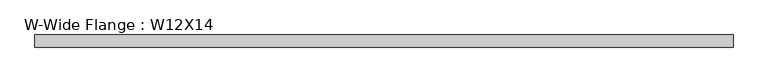
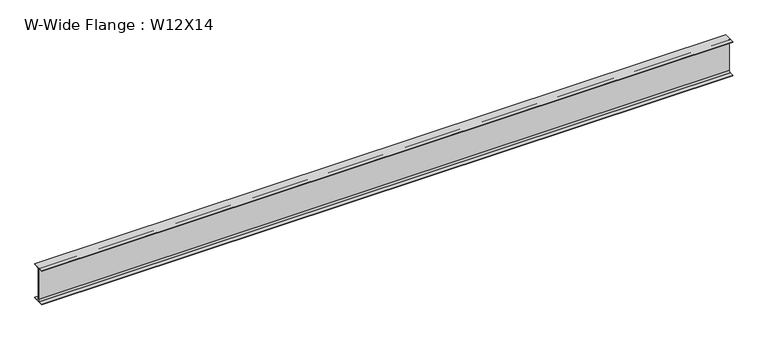
"""IFC4 building model written with IfcOpenShell, lengths in millimetres: beam geometry, W-Wide Flange : W12X14."""

import ifcopenshell
import ifcopenshell.guid

model = None  # the IFC model being written
_history = None  # IfcOwnerHistory: only IFC2X3 demands one
_inside = {}  # id of a spatial element -> (the spatial element, [elements in it])
_under = {}  # id of a project, library or spatial element -> (it, [spatial elements below it])
_declared = {}  # id of a project -> (the project, [libraries it declares])
_typed = {}  # id of a type object -> (the type object, [elements of that type])
_made_of = {}  # id of a material, layer set ... -> (it, [elements and type objects made of it])


def new_model(schema):
    """Start an empty IFC model of exactly this schema.

    Asked for "IFC4X3", IfcOpenShell would pick the latest addendum, in which some entities
    have other attributes; the version numbers below select the first issue.
    IFC2X3 requires an IfcOwnerHistory on every rooted entity: one is made here for all.
    """
    global model, _history
    if schema == "IFC4X3":
        model = ifcopenshell.file(schema_version=(4, 3, 0, 0))
    else:
        model = ifcopenshell.file(schema=schema)
    _inside.clear()
    _under.clear()
    _declared.clear()
    _typed.clear()
    _made_of.clear()
    _history = None
    if model.schema == "IFC2X3":
        org = make("IfcOrganization", Name="unknown")
        user = make(
            "IfcPersonAndOrganization",
            ThePerson=make("IfcPerson", FamilyName="unknown"),
            TheOrganization=org,
        )
        app = make(
            "IfcApplication",
            ApplicationDeveloper=org,
            Version="unknown",
            ApplicationFullName="unknown",
            ApplicationIdentifier="unknown",
        )
        _history = make(
            "IfcOwnerHistory",
            OwningUser=user,
            OwningApplication=app,
            ChangeAction="ADDED",
            CreationDate=0,
        )
    return model


def make(cls, **values):
    """One entity of the class cls with the attributes given. An attribute that is None is left unset."""
    return model.create_entity(
        cls, **{name: value for name, value in values.items() if value is not None}
    )


def rooted(cls, **values):
    """An entity with a GlobalId (a new one), such as an element, a storey or a relation."""
    return make(cls, GlobalId=ifcopenshell.guid.new(), OwnerHistory=_history, **values)


def si_unit(unit_type, name, prefix=None):
    """IfcSIUnit, for example si_unit("LENGTHUNIT", "METRE", prefix="MILLI")."""
    return make("IfcSIUnit", UnitType=unit_type, Prefix=prefix, Name=name)


def assignment(units):
    """IfcUnitAssignment: the units of a project."""
    return None if units is None else make("IfcUnitAssignment", Units=units)


def point(xyz):
    """IfcCartesianPoint."""
    return None if xyz is None else make("IfcCartesianPoint", Coordinates=xyz)


def direction(xyz):
    """IfcDirection."""
    return None if xyz is None else make("IfcDirection", DirectionRatios=xyz)


def frame(location, z_axis=None, x_axis=None):
    """IfcAxis2Placement3D, a coordinate frame: its origin and axes. An axis left out is left unset."""
    return make(
        "IfcAxis2Placement3D",
        Location=point(location),
        Axis=direction(z_axis),
        RefDirection=direction(x_axis),
    )


def frame_2d(location, x_axis=None):
    """IfcAxis2Placement2D, a coordinate frame in the plane: its origin and x axis."""
    return make(
        "IfcAxis2Placement2D", Location=point(location), RefDirection=direction(x_axis)
    )


def origin():
    """The frame at (0, 0, 0) with its axes left unset."""
    return frame((0.0, 0.0, 0.0))


def place(relative_to, where):
    """IfcLocalPlacement: puts the frame where relative to a parent placement (None: the world)."""
    return make(
        "IfcLocalPlacement", PlacementRelTo=relative_to, RelativePlacement=where
    )


def context(
    kind, dimensions, precision=None, world=None, true_north=None, identifier=None
):
    """IfcGeometricRepresentationContext, for example the 3D "Model" context."""
    return make(
        "IfcGeometricRepresentationContext",
        ContextIdentifier=identifier,
        ContextType=kind,
        CoordinateSpaceDimension=dimensions,
        Precision=precision,
        WorldCoordinateSystem=world,
        TrueNorth=true_north,
    )


def project(units=None, contexts=None):
    """IfcProject with its units and contexts."""
    return rooted(
        "IfcProject",
        Name="project",
        RepresentationContexts=contexts,
        UnitsInContext=assignment(units),
    )


def spatial(cls, under=None, at=None, **own):
    """A site, building, storey or space (cls), placed at a placement, below another one or the project."""
    s = rooted(cls, ObjectPlacement=at, **own)
    if under is not None:
        _under.setdefault(under.id(), (under, []))[1].append(s)
    return s


def polyline(points):
    """IfcPolyline through the points."""
    return make("IfcPolyline", Points=[point(p) for p in points])


def circle_curve(where, radius):
    """IfcCircle in the frame where."""
    return make("IfcCircle", Position=where, Radius=radius)


def trimmed(basis, trim1, trim2, sense, master):
    """IfcTrimmedCurve: the piece of a basis curve between two trims."""
    return make(
        "IfcTrimmedCurve",
        BasisCurve=basis,
        Trim1=trim1,
        Trim2=trim2,
        SenseAgreement=sense,
        MasterRepresentation=master,
    )


def segment(curve, same_sense, transition):
    """IfcCompositeCurveSegment."""
    return make(
        "IfcCompositeCurveSegment",
        Transition=transition,
        SameSense=same_sense,
        ParentCurve=curve,
    )


def composite_curve(segments, self_intersect=None):
    """IfcCompositeCurve: segments joined end to end."""
    return make("IfcCompositeCurve", Segments=segments, SelfIntersect=self_intersect)


def outline(outer, holes=None, kind="AREA"):
    """IfcArbitraryClosedProfileDef: a profile drawn as a closed curve; with holes, ...WithVoids."""
    if holes is None:
        return make("IfcArbitraryClosedProfileDef", ProfileType=kind, OuterCurve=outer)
    return make(
        "IfcArbitraryProfileDefWithVoids",
        ProfileType=kind,
        OuterCurve=outer,
        InnerCurves=holes,
    )


def extrude(swept, where, along, depth):
    """IfcExtrudedAreaSolid: the profile swept, set in the frame where, extruded along a direction by depth."""
    return make(
        "IfcExtrudedAreaSolid",
        SweptArea=swept,
        Position=where,
        ExtrudedDirection=direction(along),
        Depth=depth,
    )


def shape(context_of_items, identifier, shape_type, items):
    """IfcShapeRepresentation: the items that make up one representation, for example the "Body"."""
    return make(
        "IfcShapeRepresentation",
        ContextOfItems=context_of_items,
        RepresentationIdentifier=identifier,
        RepresentationType=shape_type,
        Items=items,
    )


def source(mapping_origin, context_of_items, identifier, shape_type, items):
    """IfcRepresentationMap: a shape defined once, which mapped items show again and again."""
    return make(
        "IfcRepresentationMap",
        MappingOrigin=mapping_origin,
        MappedRepresentation=shape(context_of_items, identifier, shape_type, items),
    )


def transform(
    local_origin,
    x_axis=None,
    y_axis=None,
    z_axis=None,
    scale=None,
    scale2=None,
    scale3=None,
    uniform=True,
):
    """IfcCartesianTransformationOperator3D, or its non-uniform kind. x_axis, y_axis, z_axis: its Axis1, 2, 3."""
    if uniform:
        return make(
            "IfcCartesianTransformationOperator3D",
            Axis1=direction(x_axis),
            Axis2=direction(y_axis),
            LocalOrigin=point(local_origin),
            Scale=scale,
            Axis3=direction(z_axis),
        )
    return make(
        "IfcCartesianTransformationOperator3DnonUniform",
        Axis1=direction(x_axis),
        Axis2=direction(y_axis),
        LocalOrigin=point(local_origin),
        Scale=scale,
        Axis3=direction(z_axis),
        Scale2=scale2,
        Scale3=scale3,
    )


def mapped(mapping_source, mapping_target):
    """IfcMappedItem: shows the shape of a source again, moved by a transform."""
    return make(
        "IfcMappedItem", MappingSource=mapping_source, MappingTarget=mapping_target
    )


def made_of(thing, what):
    """Note that an element or type object is made of a material, layer set ...; save() writes the relation."""
    if what is not None:
        _made_of.setdefault(what.id(), (what, []))[1].append(thing)
    return thing


def element(
    cls,
    number,
    at=None,
    inside=None,
    cuts=None,
    type_object=None,
    material=None,
    context=None,
    identifier="Body",
    shape_type=None,
    held_by="IfcProductDefinitionShape",
    body=None,
    shapes=None,
    **own,
):
    """One element of the class cls, such as IfcWall. Its Tag is "e" and its number.

    at: its placement. inside: the storey or other place that contains it. cuts: it is an
    opening in that element (IfcRelVoidsElement). A single representation is given by context,
    identifier, shape_type and body (its items); several are given by shapes. held_by: the class
    of the entity that holds the representations. save() writes the other relations.
    """
    e = rooted(cls, Tag="e%d" % number, ObjectPlacement=at, **own)
    if body is not None:
        shapes = [shape(context, identifier, shape_type, body)]
    if shapes is not None:
        e.Representation = make(held_by, Representations=shapes)
    if inside is not None:
        _inside.setdefault(inside.id(), (inside, []))[1].append(e)
    if cuts is not None:
        rooted(
            "IfcRelVoidsElement", RelatingBuildingElement=cuts, RelatedOpeningElement=e
        )
    if type_object is not None:
        _typed.setdefault(type_object.id(), (type_object, []))[1].append(e)
    return made_of(e, material)


def aggregate(whole, parts):
    """IfcRelAggregates: a whole, such as a stair, and the parts it consists of."""
    return rooted("IfcRelAggregates", RelatingObject=whole, RelatedObjects=parts)


def save(model, path):
    """Write the relations noted so far, then the file.

    IfcRelAggregates (storeys below a building ...), IfcRelContainedInSpatialStructure (elements
    in a storey), IfcRelDefinesByType, IfcRelAssociatesMaterial and IfcRelDeclares: one each for
    every whole, place, type object, material and project.
    """
    for whole, parts in _under.values():
        aggregate(whole, parts)
    for where, things in _inside.values():
        rooted(
            "IfcRelContainedInSpatialStructure",
            RelatedElements=things,
            RelatingStructure=where,
        )
    for kind, things in _typed.values():
        rooted("IfcRelDefinesByType", RelatedObjects=things, RelatingType=kind)
    for what, things in _made_of.values():
        rooted("IfcRelAssociatesMaterial", RelatedObjects=things, RelatingMaterial=what)
    for by, libraries in _declared.values():
        rooted("IfcRelDeclares", RelatingContext=by, RelatedDefinitions=libraries)
    model.write(path)


def w_wide_flange_w12x14_2a641178(model_context):
    return source(origin(), model_context, "Body", "SweptSolid", [
        extrude(outline(composite_curve([segment(polyline([(50.419, -145.415), (50.419, -151.13), (-50.419, -151.13), (-50.419, -145.415), (-15.875, -145.415)]), True, "CONTINUOUS"), segment(trimmed(circle_curve(frame_2d((-15.875, -132.08)), 13.335), [point((-15.875, -145.415))], [point((-2.54, -132.08))], True, "CARTESIAN"), True, "CONTINUOUS"), segment(polyline([(-2.54, -132.08), (-2.54, 132.08)]), True, "CONTINUOUS"), segment(trimmed(circle_curve(frame_2d((-15.875, 132.08)), 13.335), [point((-2.54, 132.08))], [point((-15.875, 145.415))], True, "CARTESIAN"), True, "CONTINUOUS"), segment(polyline([(-15.875, 145.415), (-50.419, 145.415), (-50.419, 151.13), (50.419, 151.13), (50.419, 145.415), (15.875, 145.415)]), True, "CONTINUOUS"), segment(trimmed(circle_curve(frame_2d((15.875, 132.08)), 13.335), [point((15.875, 145.415))], [point((2.54, 132.08))], True, "CARTESIAN"), True, "CONTINUOUS"), segment(polyline([(2.54, 132.08), (2.54, -132.08)]), True, "CONTINUOUS"), segment(trimmed(circle_curve(frame_2d((15.875, -132.08)), 13.335), [point((2.54, -132.08))], [point((15.875, -145.415))], True, "CARTESIAN"), True, "CONTINUOUS"), segment(polyline([(15.875, -145.415), (50.419, -145.415)]), True, "CONTINUOUS")], self_intersect=False)), frame((-2959.1, 0.0, 0.0), z_axis=(1.0, 0.0, 0.0), x_axis=(0.0, 1.0, 0.0)), (0.0, 0.0, 1.0), 5816.6),
    ])


if __name__ == "__main__":
    model = new_model("IFC4")
    model_context = context("Model", 3, world=origin())
    ifc_project = project(units=[si_unit("LENGTHUNIT", "METRE", prefix="MILLI")], contexts=[model_context])
    site = spatial("IfcSite", under=ifc_project)
    building = spatial("IfcBuilding", under=site)
    placement = place(None, origin())
    w_wide_flange_w12x14_shape = w_wide_flange_w12x14_2a641178(model_context)
    element("IfcBeam", 1, ObjectType="W-Wide Flange : W12X14", at=placement, inside=building, context=model_context, shape_type="MappedRepresentation", body=[
        mapped(w_wide_flange_w12x14_shape, transform((0.0, 0.0, 0.0), x_axis=(1.0, 0.0, 0.0), y_axis=(0.0, 1.0, 0.0), z_axis=(0.0, 0.0, 1.0))),
    ])
    save(model, "model.ifc")

# Revit data of these elements
# Type "W-Wide Flange : W12X14"
#   Assembly Code = "B10"
#   W = 14
#   Length [instance default] = 5' - 0"
#   bf = 0' - 3.97"
#   d = 0' - 11.9"
#   k = 0' - 0 3/4"
#   k2 = 0' - 0.525"
#   tf = 0' - 0.225"
#   tw = 0' - 0.2"
#   A = 0.0288889 SF
#   Structural Material [instance default] = Steel ASTM A992
# Element 1 (IfcBeam, "W-Wide Flange : W12X14")
#   Materials on its faces: "Steel ASTM A992"
# Materials
#   "Steel ASTM A992": class "Metal", colour RGB 199 199 199, transparency 0, Description = "Structural steel 50ksi", Cost = 0
